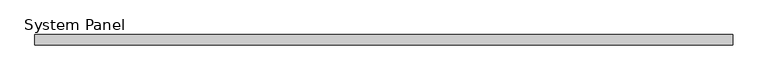
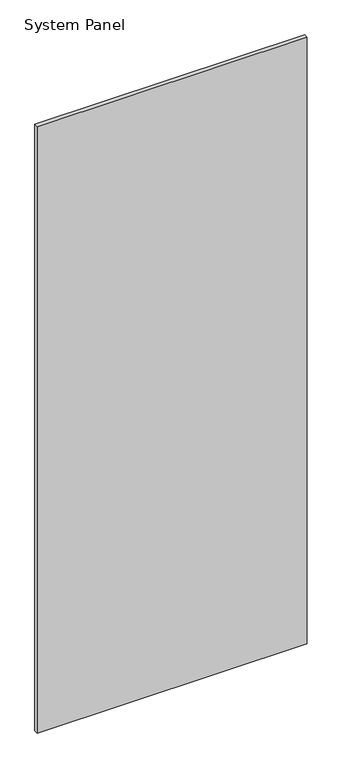
"""IFC4 building model written with IfcOpenShell, lengths in millimetres: plate geometry, System Panel : WWm-Glass-20mm-10mmOffset."""

from ifc_helpers import new_model, si_unit, origin, origin_with_axes, place, context, project, spatial, polyline, outline, extrude, source, transform, mapped, element, save


def system_panel_289df84f(model_context):
    return source(origin(), model_context, "Body", "SweptSolid", [
        extrude(outline(polyline([(685.0, 0.0), (-685.0, 0.0), (-685.0, 20.0), (685.0, 20.0), (685.0, 0.0)])), origin_with_axes(), (0.0, 0.0, 1.0), 3250.0),
    ])


if __name__ == "__main__":
    model = new_model("IFC4")
    model_context = context("Model", 3, world=origin())
    ifc_project = project(units=[si_unit("LENGTHUNIT", "METRE", prefix="MILLI")], contexts=[model_context])
    site = spatial("IfcSite", under=ifc_project)
    building = spatial("IfcBuilding", under=site)
    placement = place(None, origin())
    system_panel_shape = system_panel_289df84f(model_context)
    element("IfcPlate", 1, ObjectType="System Panel : WWm-Glass-20mm-10mmOffset", at=placement, inside=building, context=model_context, shape_type="MappedRepresentation", body=[
        mapped(system_panel_shape, transform((0.0, 0.0, 0.0), x_axis=(1.0, 0.0, 0.0), y_axis=(0.0, 1.0, 0.0), z_axis=(0.0, 0.0, 1.0))),
    ])
    save(model, "model.ifc")

# Revit data of these elements
# Type "System Panel : WWm-Glass-20mm-10mmOffset"
#   Finish = ""
# Element 1 (IfcPlate, "System Panel : WWm-Glass-20mm-10mmOffset")
#   Materials on its faces: "WW-EC-GL-Storefront"
# Materials
#   "WW-EC-GL-Storefront": class "Glass", colour RGB 236 240 239, transparency 0.85, Description = "Storefront Glass", Cost = 0
